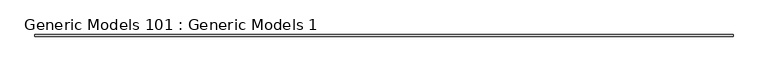
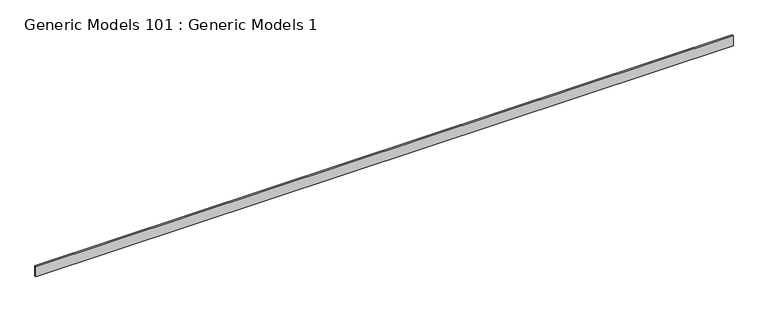
"""IFC4 building model written with IfcOpenShell, lengths in millimetres: proxy geometry, Generic Models 101 : Generic Models 1."""

from ifc_helpers import new_model, si_unit, frame, origin, place, context, project, spatial, polyline, outline, extrude, source, transform, mapped, element, save


def generic_models_101_generic_models_1_6d181150(model_context):
    return source(origin(), model_context, "Body", "SweptSolid", [
        extrude(outline(polyline([(-20998.9733045, 51294.7476718), (-20998.9733045, 51339.1976718), (-1948.9733045, 51339.1976718), (-1948.9733045, 51294.7476718), (-20998.9733045, 51294.7476718)])), frame((0.0, 0.0, 126523.496), z_axis=(0.0, 0.0, 1.0), x_axis=(1.0, 0.0, 0.0)), (0.0, 0.0, 1.0), 285.75),
    ])


if __name__ == "__main__":
    model = new_model("IFC4")
    model_context = context("Model", 3, world=origin())
    ifc_project = project(units=[si_unit("LENGTHUNIT", "METRE", prefix="MILLI")], contexts=[model_context])
    site = spatial("IfcSite", under=ifc_project)
    building = spatial("IfcBuilding", under=site)
    placement = place(None, origin())
    generic_models_101_generic_models_1_shape = generic_models_101_generic_models_1_6d181150(model_context)
    element("IfcBuildingElementProxy", 1, Name="Generic Models 101 : Generic Models 1", ObjectType="Generic Models 101 : Generic Models 1", at=placement, inside=building, context=model_context, shape_type="MappedRepresentation", body=[
        mapped(generic_models_101_generic_models_1_shape, transform((0.0, 0.0, 0.0), x_axis=(1.0, 0.0, 0.0), y_axis=(0.0, 1.0, 0.0), z_axis=(0.0, 0.0, 1.0))),
    ])
    save(model, "model.ifc")

# Revit data of these elements
# Element 1 (IfcBuildingElementProxy, "Generic Models 101 : Generic Models 1")
#   Materials on its faces: "_STRUCTURAL MEMBER (SEE STRUCT. DWGS)"
# Materials
#   "_STRUCTURAL MEMBER (SEE STRUCT. DWGS)": class "Generic", colour RGB 209 182 141, transparency 0, Cost = 0
